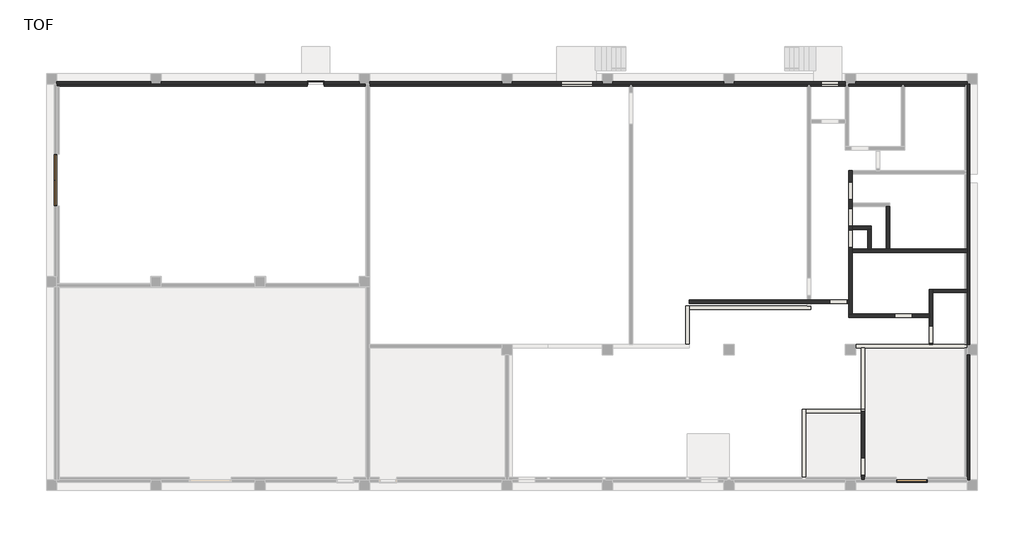
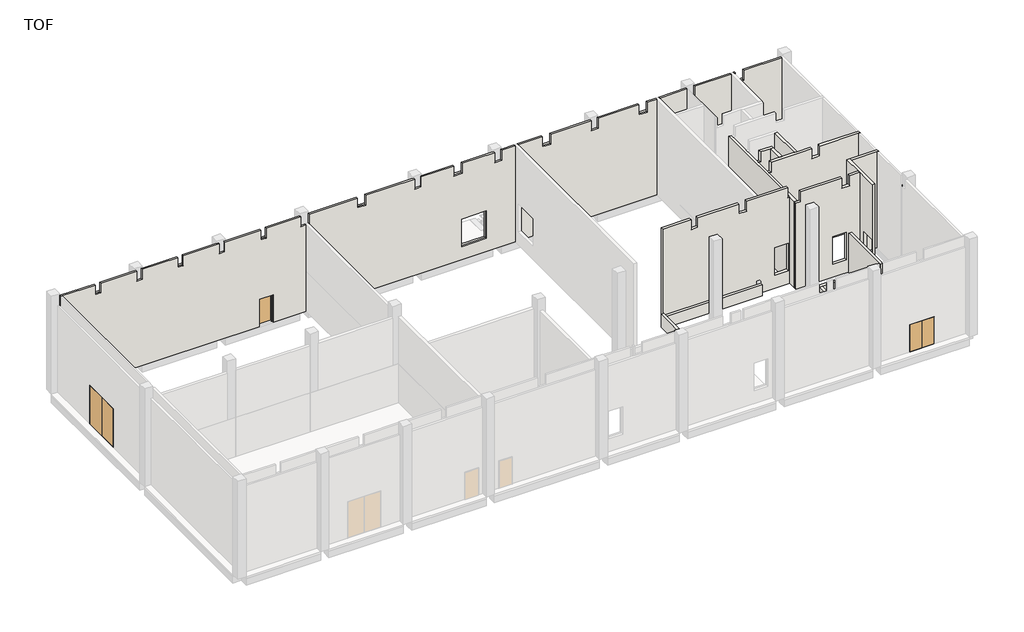
# One storey, part 2 of 4: 19 walls, 3 doors.
# Revit data of these elements (continued)
# Type "Double Door_Steel : H_DR_AR_B12_Double Door_Steel_W2000xH2100" (continued)
#   문번호 = ""
#   문기호 = "SD"
#   Analytic Construction = "<None>"
#   Height = 2100 mm
#   Width = 1800 mm
#   Define Thermal Properties by = 1
#   문 틀 = none
#   문 = none
#   Function = (empty or 0)
#   Assembly Code = ""
#   Wall Closure = (empty or 0)
# Type "Double Door_Steel : H_DR_AR_B12_Double Door_Steel_W3000xH3000"
#   Type Mark = "430"
#   프레임 = ""
#   철물 = ""
#   유리/마감 = ""
#   위치/개소 = ""
#   부호 = "1/SD"
#   문번호 = ""
#   문기호 = "SD"
#   Analytic Construction = "<None>"
#   Height = 3000 mm
#   Width = 3000 mm
#   Define Thermal Properties by = 1
#   문 틀 = none
#   문 = none
#   Function = (empty or 0)
#   Assembly Code = ""
#   Wall Closure = (empty or 0)
# Type "Single Door_Steel : H_DR_AR_B12_Single Door_Steel_W1000xH2100"
#   Type Mark = "SD"
#   Analytic Construction = "<None>"
#   프레임 투영 외부. = 25 mm
#   프레임 투영 내부. = 25 mm
#   프레임 폭 = 75 mm
#   Height = 2100 mm
#   Width = 1000 mm
#   Define Thermal Properties by = 1
#   문 패널 = none
#   문 프레임 = none
#   Function = (empty or 0)
#   Wall Closure = (empty or 0)
# Type "H_WA_AR_B02_Ext Wall_RC T150"
#   Type Comments = ""
#   Layers, outside or top first: 150 mm "Concrete - Cast-in-Place Concrete - 35 MPa" (function 1)
# Type "H_WA_AR_B02_Int Wall_Block T200"
#   Type Comments = ""
#   Layers, outside or top first: 200 mm "00_Masonry_Conc. Block" (function 1)
# Type "H_WA_AR_B02_Ext Wall_1L Gypsum_Mineral Wool_T110"
#   Type Comments = "구조_콘크리트"
#   Layers, outside or top first: 110 mm "Rock Wool" (function 2); 16 mm "Gypsum Wall Board" (function 1)
# Type "H_WA_AR_B02_Int Wall_RC"
#   Type Comments = ""
#   Layers, outside or top first: 200 mm "Concrete - Cast-in-Place Concrete - 35 MPa" (function 1)
# Element 1 (IfcDoor, "Double Door_Steel : H_DR_AR_B12_Double Door_Steel_W2000xH2100")
#   H_Door Style Name = "Steel Door_Double"
#   H_Door_Frame = "Steel"
#   H_Door_Leaf = "Steel"
#   H_Door_Vision = "N.A"
#   H_Door_Panic = "N.A"
#   H_Door_Style Remark = ""
#   H_Door_Fire Rating = "NA/0.5/1.0\n/1.5/2.0"
#   H_Door Style No = DD11
#   Phase Created = New Construction
# Element 2 (IfcDoor, "Double Door_Steel : H_DR_AR_B12_Double Door_Steel_W3000xH3000")
#   H_Door Style Name = "Steel Door_Double_Transsom"
#   H_Door_Frame = "Steel"
#   H_Door_Leaf = "Steel"
#   H_Door_Vision = "N.A"
#   H_Door_Panic = "N.A"
#   H_Door_Style Remark = ""
#   H_Door_Fire Rating = "NA/0.5/1.0\n/1.5/2.0"
#   H_Door Style No = DDT11
#   Phase Created = New Construction
# Element 3 (IfcDoor, "Single Door_Steel : H_DR_AR_B12_Single Door_Steel_W1000xH2100")
#   H_Door Style Name = "Steel Door_Single"
#   H_Door_Frame = "Steel"
#   H_Door_Leaf = "Steel"
#   H_Door_Vision = "N.A"
#   H_Door_Panic = "N.A"
#   H_Door_Style Remark = "Steel Door w/ Steel Frame"
#   H_Door_Fire Rating = "NA/0.5/1.0\n/1.5/2.0"
#   H_Door Style No = SD11
#   Phase Created = New Construction
# Elements 4, 5 (IfcWall, "H_WA_AR_B02_Ext Wall_RC T150")
#   H_Wall Style Name = "Gypsum Board Wall+Mineral Wool Insulation w/ Air Space+Concrete Wall+Acrylic Emulsion Paint on Fair Faced Concrete"
#   H_Wall-Base Material-1 = "1-Layer Gypsum Board"
#   H_Wall-Base Material-2 = "Mineral Wool (Rock Wool)+Air Space"
#   H_Wall_Finish-In = "Acrylic Emulsion Paint"
#   H_Wall_Base Material-3 = "Concrete Wall"
#   H_Wall_Finish-Ex = "Acrylic Emulsion Paint on Fair Faced Concrete"
#   H_Wall_Style Remark = "WM : Plasterboard Dry Liner System (A04AS176-00001~00009)\n        - Gypsum Board + Insulation\n        (Gypsumboard THK=9.5 & 12.5 & 16 mm)"
#   Top Offset = 0 mm
#   Base Offset = 0 mm
#   wall height = 7500 mm
#   H_Wall Style No = EW11
#   Phase Created = New Construction
#   Base Constraint = TOF
#   Top Constraint = TOC
#   Materials on its faces: "Concrete - Cast-in-Place Concrete - 35 MPa"
# Elements 6, 8, 9, 10, 11, 12, 13, 14, 15 (IfcWall, "H_WA_AR_B02_Int Wall_Block T200")
#   H_Wall Style Name = "Block Wall"
#   H_Wall-Base Material-1 = "Concrete Block"
#   H_Wall-Base Material-2 = ""
#   H_Wall_Finish-In = "Acrylic Emulsion Paint on Cement Plaster"
#   H_Wall_Base Material-3 = ""
#   H_Wall_Finish-Ex = "Acrylic Emulsion Paint on Cement Plaster"
#   H_Wall_Style Remark = "WM : Reinforced Concrete Block\n     50mm<THK≤100mm / 100mm<THK≤200mm / 200mm<THK"
#   Top Offset = 0 mm
#   Base Offset = 0 mm
#   wall height = 7500 mm
#   H_Wall Style No = IW21
#   Phase Created = New Construction
#   Base Constraint = TOF
#   Top Constraint = TOC
#   Materials on its faces: "00_Masonry_Conc. Block"
# Element 7 (IfcWall, "H_WA_AR_B02_Int Wall_Block T200")
#   H_Wall Style Name = "Block Wall"
#   H_Wall-Base Material-1 = "Concrete Block"
#   H_Wall-Base Material-2 = ""
#   H_Wall_Finish-In = "Acrylic Emulsion Paint on Cement Plaster"
#   H_Wall_Base Material-3 = ""
#   H_Wall_Finish-Ex = "Acrylic Emulsion Paint on Cement Plaster"
#   H_Wall_Style Remark = "WM : Reinforced Concrete Block\n     50mm<THK≤100mm / 100mm<THK≤200mm / 200mm<THK"
#   Top Offset = 0 mm
#   Base Offset = 0 mm
#   wall height = 7500 mm
#   H_Wall Style No = IW21
#   Phase Created = New Construction
#   Base Constraint = TOF
#   Top Constraint = TOC
#   Materials on its faces: "00_Masonry_Conc. Block", "Concrete - Cast-in-Place Concrete - 35 MPa"
# Element 16 (IfcWall, "H_WA_AR_B02_Ext Wall_1L Gypsum_Mineral Wool_T110")
#   Top Offset = 0 mm
#   Base Offset = 0 mm
#   wall height = 7500 mm
#   Phase Created = New Construction
#   Base Constraint = TOF
#   Top Constraint = TOC
#   Materials on its faces: "Rock Wool", "Gypsum Wall Board"
# Elements 17, 18, 19, 20, 21, 22 (IfcWall, "H_WA_AR_B02_Int Wall_RC")
#   Top Offset = 0 mm
#   Base Offset = 0 mm
#   wall height = 1000 mm
#   Phase Created = New Construction
#   Base Constraint = TOF
#   Top Constraint = TOF2
#   Materials on its faces: "Concrete - Cast-in-Place Concrete - 35 MPa"
# Materials
#   "Concrete - Cast-in-Place Concrete - 35 MPa": class "Concrete", colour RGB 192 192 192, transparency 0, Cost = 0
#   "00_Masonry_Conc. Block": class "Concrete", colour RGB 180 180 180, transparency 0, Description = "Conc. Block", Cost = 0, Image = Brick_Uniform_12inch_Running_Gray.png
#   "Rock Wool": class "Generic", colour RGB 120 120 120, transparency 0, Description = "Rock Wool", Cost = 0
#   "Gypsum Wall Board": class "Generic", colour RGB 171 170 168, transparency 0, Description = "Gypsum Wall Board", Cost = 0
